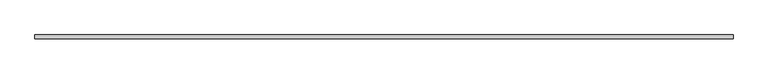
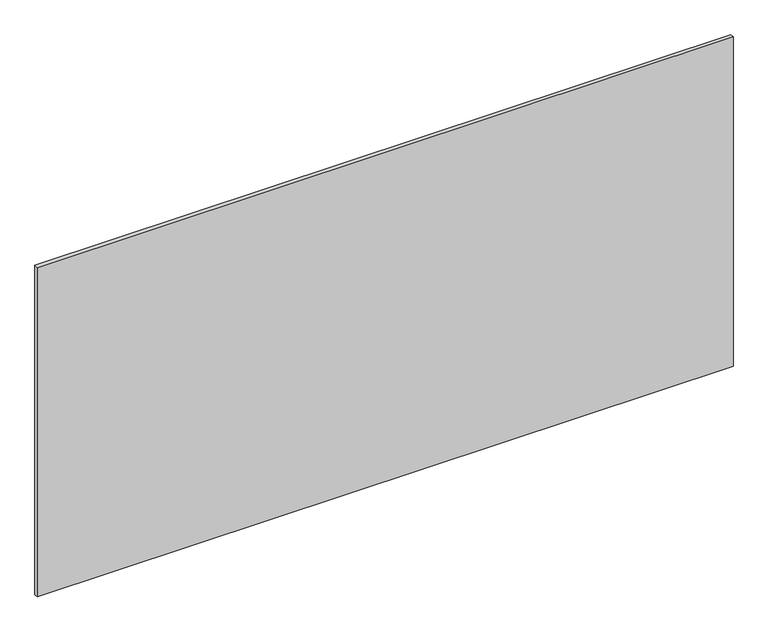
"""IFC4 building model written with IfcOpenShell, lengths in millimetres: proxy geometry, Inner panel:Inner panel:1:Inner panel:1 : Inner panel:Inner panel:300324:300043:Inner panel:1:Inner panel:1 : Inner panel:Inner panel:300324:300043 : Inner panel:Inner panel:1:Inner panel:1 : Inner panel:Inner panel:300324:300043:9 : Inner panel:Inner panel:1:Inner panel:1 : Inner panel:Inner panel:300324:300043:Inner panel:1:Inner panel:1 : Inner panel:Inner panel:300324:300043 : Inner panel:Inner panel:1:Inner panel:1 : Inner panel:Inner panel:300324:300043:300031."""

from ifc_helpers import new_model, si_unit, frame, origin, place, context, project, spatial, polyline, outline, extrude, source, transform, mapped, element, save


def generic_models_074a640e(model_context):
    return source(origin(), model_context, "Body", "SweptSolid", [
        extrude(outline(polyline([(570452.6367239, -579000.6913841), (572891.0367239, -579000.6913841), (572891.0367239, -579013.3913841), (570452.6367239, -579013.3913841), (570452.6367239, -579000.6913841)])), frame((0.0, 0.0, 3721.1), z_axis=(0.0, 0.0, 1.0), x_axis=(1.0, 0.0, 0.0)), (0.0, 0.0, 1.0), 1219.2),
    ])


if __name__ == "__main__":
    model = new_model("IFC4")
    model_context = context("Model", 3, world=origin())
    ifc_project = project(units=[si_unit("LENGTHUNIT", "METRE", prefix="MILLI")], contexts=[model_context])
    site = spatial("IfcSite", under=ifc_project)
    building = spatial("IfcBuilding", under=site)
    placement = place(None, origin())
    generic_models_shape = generic_models_074a640e(model_context)
    element("IfcBuildingElementProxy", 1, Name="Inner panel:Inner panel:1:Inner panel:1 : Inner panel:Inner panel:300324:300043:Inner panel:1:Inner panel:1 : Inner panel:Inner panel:300324:300043 : Inner panel:Inner panel:1:Inner panel:1 : Inner panel:Inner panel:300324:300043:9 : Inner panel:Inner panel:1:Inner panel:1 : Inner panel:Inner panel:300324:300043:Inner panel:1:Inner panel:1 : Inner panel:Inner panel:300324:300043 : Inner panel:Inner panel:1:Inner panel:1 : Inner panel:Inner panel:300324:300043:300031", ObjectType="Inner panel:Inner panel:1:Inner panel:1 : Inner panel:Inner panel:300324:300043:Inner panel:1:Inner panel:1 : Inner panel:Inner panel:300324:300043 : Inner panel:Inner panel:1:Inner panel:1 : Inner panel:Inner panel:300324:300043:9 : Inner panel:Inner panel:1:Inner panel:1 : Inner panel:Inner panel:300324:300043:Inner panel:1:Inner panel:1 : Inner panel:Inner panel:300324:300043 : Inner panel:Inner panel:1:Inner panel:1 : Inner panel:Inner panel:300324:300043:300031", at=placement, inside=building, context=model_context, shape_type="MappedRepresentation", body=[
        mapped(generic_models_shape, transform((0.0, 0.0, 0.0), x_axis=(1.0, 0.0, 0.0), y_axis=(0.0, 1.0, 0.0), z_axis=(0.0, 0.0, 1.0))),
    ])
    save(model, "model.ifc")

# Revit data of these elements
# Type "Inner panel:Inner panel:1:Inner panel:1 : Inner panel:Inner panel:300324:300043:Inner panel:1:Inner panel:1 : Inner panel:Inner panel:300324:300043 : Inner panel:Inner panel:1:Inner panel:1 : Inner panel:Inner panel:300324:300043:9 : Inner panel:Inner panel:1:Inner panel:1 : Inner panel:Inner panel:300324:300043:Inner panel:1:Inner panel:1 : Inner panel:Inner panel:300324:300043 : Inner panel:Inner panel:1:Inner panel:1 : Inner panel:Inner panel:300324:300043:300031"
#   NameOverride = "Inner panel:Inner panel:1:Inner panel:1 : Inner panel:Inner panel:300324:300043:Inner panel:1:Inner panel:1 : Inner panel:Inner panel:300324:300043 : Inner panel:Inner panel:1:Inner panel:1 : Inner panel:Inner panel:300324:300043:300031"
#   ObjectTypeOverride = "Inner panel:1:Inner panel:1 : Inner panel:Inner panel:300324:300043 : Inner panel:Inner panel:1:Inner panel:1 : Inner panel:Inner panel:300324:300043"
#   Reference = "Inner panel"
#   Tag = "300031"
# Element 1 (IfcBuildingElementProxy, "Inner panel:Inner panel:1:Inner panel:1 : Inner panel:Inner panel:300324:300043:Inner panel:1:Inner panel:1 : Inner panel:Inner panel:300324:300043 : Inner panel:Inner panel:1:Inner panel:1 : Inner panel:Inner panel:300324:300043:9 : Inner panel:Inner panel:1:Inner panel:1 : Inner panel:Inner panel:300324:300043:Inner panel:1:Inner panel:1 : Inner panel:Inner panel:300324:300043 : Inner panel:Inner panel:1:Inner panel:1 : Inner panel:Inner panel:300324:300043:300031")
#   Materials on its faces: "1/2\" EXTERIOR GRADE FIRE RETARDANT CDX PLYWOOD"
# Materials
#   "1/2\" EXTERIOR GRADE FIRE RETARDANT CDX PLYWOOD": class "Unassigned", colour RGB 196 177 123, transparency 0, Cost = 0
